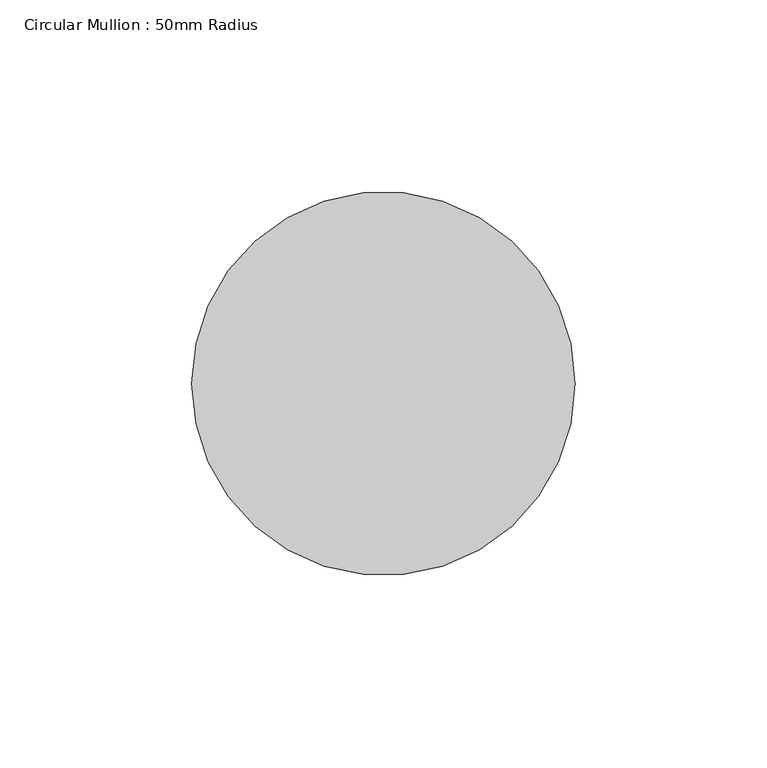
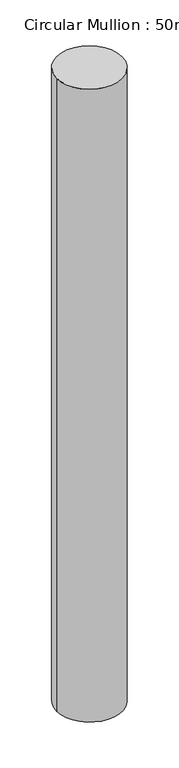
"""IFC4 building model written with IfcOpenShell, lengths in millimetres: member geometry, Circular Mullion : 50mm Radius."""

from ifc_helpers import new_model, si_unit, point, frame, origin, origin_2d, place, context, project, spatial, circle_curve, trimmed, segment, composite_curve, outline, extrude, source, transform, mapped, element, save


def circular_mullion_50mm_radius_b156845f(model_context):
    return source(origin(), model_context, "Body", "SweptSolid", [
        extrude(outline(composite_curve([segment(trimmed(circle_curve(origin_2d(), 50.0), [point((50.0, 0.0))], [point((-50.0, 0.0))], False, "CARTESIAN"), True, "CONTINUOUS"), segment(trimmed(circle_curve(origin_2d(), 50.0), [point((-50.0, 0.0))], [point((50.0, 0.0))], False, "CARTESIAN"), True, "CONTINUOUS")], self_intersect=False)), frame((0.0, 0.0, -1020.1783803), z_axis=(0.0, 0.0, 1.0), x_axis=(1.0, 0.0, 0.0)), (0.0, 0.0, 1.0), 1020.1783803),
    ])


if __name__ == "__main__":
    model = new_model("IFC4")
    model_context = context("Model", 3, world=origin())
    ifc_project = project(units=[si_unit("LENGTHUNIT", "METRE", prefix="MILLI")], contexts=[model_context])
    site = spatial("IfcSite", under=ifc_project)
    building = spatial("IfcBuilding", under=site)
    placement = place(None, origin())
    circular_mullion_50mm_radius_shape = circular_mullion_50mm_radius_b156845f(model_context)
    element("IfcMember", 1, ObjectType="Circular Mullion : 50mm Radius", at=placement, inside=building, context=model_context, shape_type="MappedRepresentation", body=[
        mapped(circular_mullion_50mm_radius_shape, transform((0.0, 0.0, 0.0), x_axis=(1.0, 0.0, 0.0), y_axis=(0.0, 1.0, 0.0), z_axis=(0.0, 0.0, 1.0))),
    ])
    save(model, "model.ifc")

# Revit data of these elements
# Type "Circular Mullion : 50mm Radius"
#   built-in parameter 1007350 = 0.164042 (stored number, unit not read)
# Element 1 (IfcMember, "Circular Mullion : 50mm Radius")
#   Materials on its faces: "Aluminium"
# Materials
#   "Aluminium": class "Metal", colour RGB 247 247 247, transparency 0, Description = "Aluminium 6061", Cost = 0
